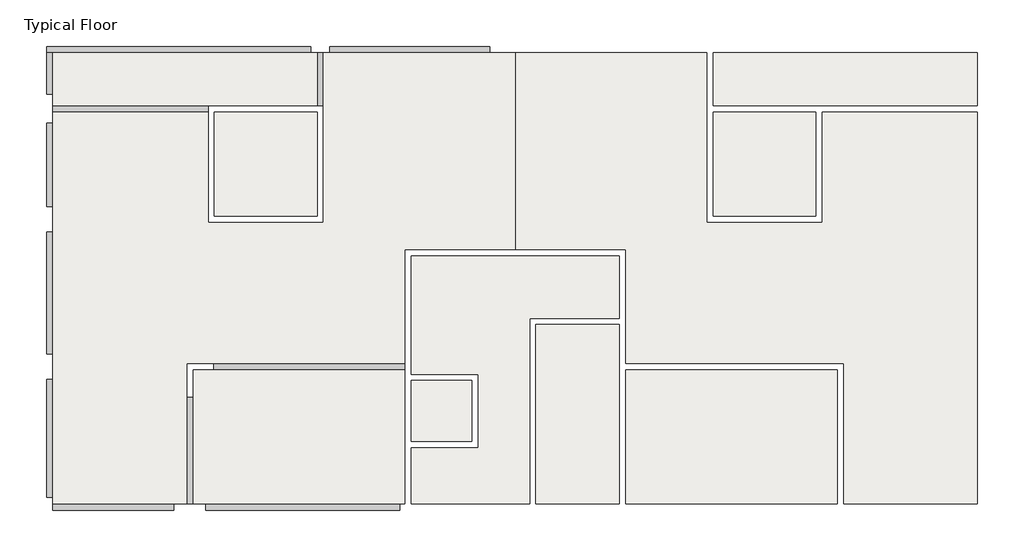
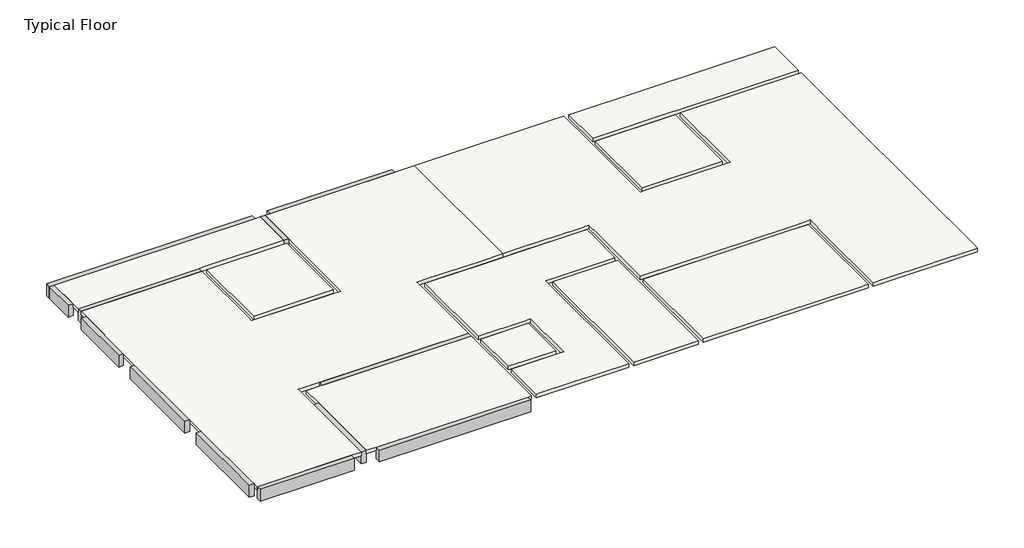
# One storey: 12 beams, 11 slabs.
"""IFC4 building model written with IfcOpenShell, lengths in millimetres."""

from ifc_helpers import new_model, si_unit, frame, origin, place, context, project, spatial, polyline, outline, extrude, faceted_brep, element, save

model = new_model("IFC4")

# Units and contexts
model_context = context("Model", 3, world=origin())
ifc_project = project(units=[si_unit("LENGTHUNIT", "METRE", prefix="MILLI")], contexts=[model_context])

# Site, building, storey
site = spatial("IfcSite", under=ifc_project)
building = spatial("IfcBuilding", under=site)
storey = spatial("IfcBuildingStorey", under=building, Name="Typical Floor", Elevation=3000.0)

# Beams
placement = place(None, origin())
element("IfcBeam", 1, ObjectType="Concrete Rectengular Beam : 20/50", at=placement, inside=storey, context=model_context, shape_type="SweptSolid", body=[
    extrude(outline(polyline([(-9297.7826138, 4182.4555068), (-9297.7826138, 4382.4555068), (-4303.3703529, 4382.4555068), (-4303.3703529, 4182.4555068), (-9297.7826138, 4182.4555068)])), frame((0.0, 0.0, 2500.0), z_axis=(0.0, 0.0, 1.0), x_axis=(1.0, 0.0, 0.0)), (0.0, 0.0, 1.0), 500.0),
])
element("IfcBeam", 2, ObjectType="Concrete Rectengular Beam : 20/50", at=placement, inside=storey, context=model_context, shape_type="Brep", body=[
    faceted_brep([(-18150.6144474, 4382.4555068, 3000.0), (-18150.6144474, 4182.4555068, 3000.0), (-17950.6144474, 4182.4555068, 3000.0), (-9897.7826138, 4182.4555068, 3000.0), (-9897.7826138, 4382.4555068, 3000.0), (-18150.6144474, 4182.4555068, 2500.0), (-17950.6144474, 4182.4555068, 2500.0), (-9897.7826138, 4182.4555068, 2500.0), (-18150.6144474, 4382.4555068, 2500.0), (-9897.7826138, 4382.4555068, 2500.0)], [[[0, 1, 2, 3, 4]], [[1, 5, 6, 7, 3, 2]], [[5, 8, 9, 7, 6]], [[8, 0, 4, 9]], [[4, 3, 7, 9]], [[1, 0, 8, 5]]]),
])
element("IfcBeam", 3, ObjectType="Concrete Rectengular Beam : 20/50", at=placement, inside=storey, context=model_context, shape_type="Brep", body=[
    faceted_brep([(-18150.6144474, 2884.276373, 3000.0), (-17950.6144474, 2884.276373, 3000.0), (-17950.6144474, 4182.4555068, 3000.0), (-18150.6144474, 4182.4555068, 3000.0), (-17950.6144474, 2884.276373, 2500.0), (-17950.6144474, 4182.4555068, 2500.0), (-17950.6144474, 4182.4555068, 2850.0), (-18150.6144474, 2884.276373, 2500.0), (-18150.6144474, 4182.4555068, 2500.0)], [[[0, 1, 2, 3]], [[1, 4, 5, 6, 2]], [[4, 7, 8, 5]], [[7, 0, 3, 8]], [[1, 0, 7, 4]], [[3, 2, 6, 5, 8]]]),
])
element("IfcBeam", 4, ObjectType="Concrete Rectengular Beam : 20/50", at=placement, inside=storey, context=model_context, shape_type="SweptSolid", body=[
    extrude(outline(polyline([(-17950.6144474, -618.260185), (-18150.6144474, -618.260185), (-18150.6144474, 1984.276373), (-17950.6144474, 1984.276373), (-17950.6144474, -618.260185)])), frame((0.0, 0.0, 2500.0), z_axis=(0.0, 0.0, 1.0), x_axis=(1.0, 0.0, 0.0)), (0.0, 0.0, 1.0), 500.0),
])
element("IfcBeam", 5, ObjectType="Concrete Rectengular Beam : 20/50", at=placement, inside=storey, context=model_context, shape_type="SweptSolid", body=[
    extrude(outline(polyline([(-18150.6144474, -1418.260185), (-17950.6144474, -1418.260185), (-17950.6144474, -5238.12942), (-18150.6144474, -5238.12942), (-18150.6144474, -1418.260185)])), frame((0.0, 0.0, 2500.0), z_axis=(0.0, 0.0, 1.0), x_axis=(1.0, 0.0, 0.0)), (0.0, 0.0, 1.0), 500.0),
])
element("IfcBeam", 6, ObjectType="Concrete Rectengular Beam : 20/50", at=placement, inside=storey, context=model_context, shape_type="SweptSolid", body=[
    extrude(outline(polyline([(-18150.6144474, -6038.12942), (-17950.6144474, -6038.12942), (-17950.6144474, -9718.1209836), (-18150.6144474, -9718.1209836), (-18150.6144474, -6038.12942)])), frame((0.0, 0.0, 2500.0), z_axis=(0.0, 0.0, 1.0), x_axis=(1.0, 0.0, 0.0)), (0.0, 0.0, 1.0), 500.0),
])
element("IfcBeam", 7, ObjectType="Concrete Rectengular Beam : 20/50", at=placement, inside=storey, context=model_context, shape_type="Brep", body=[
    faceted_brep([(-12922.2278424, -5538.12942, 3000.0), (-12922.2278424, -5738.12942, 3000.0), (-6954.5134912, -5738.12942, 3000.0), (-6954.5134912, -5538.12942, 3000.0), (-12922.2278424, -5538.12942, 2500.0), (-12922.2278424, -5538.12942, 2850.0), (-6954.5134912, -5538.12942, 2850.0), (-6954.5134912, -5538.12942, 2500.0), (-12922.2278424, -5738.12942, 2500.0), (-6954.5134912, -5738.12942, 2500.0), (-6954.5134912, -5738.12942, 2850.0)], [[[0, 1, 2, 3]], [[4, 5, 0, 3, 6, 7]], [[8, 4, 7, 9]], [[1, 8, 9, 10, 2]], [[1, 0, 5, 4, 8]], [[3, 2, 10, 9, 7, 6]]]),
])
element("IfcBeam", 8, ObjectType="Concrete Rectengular Beam : 20/50", at=placement, inside=storey, context=model_context, shape_type="Brep", body=[
    faceted_brep([(-13772.2278424, -9918.1209836, 3000.0), (-13572.2278424, -9918.1209836, 3000.0), (-13572.2278424, -6588.12942, 3000.0), (-13772.2278424, -6588.12942, 3000.0), (-13572.2278424, -9918.1209836, 2850.0), (-13572.2278424, -9918.1209836, 2500.0), (-13572.2278424, -6588.12942, 2500.0), (-13772.2278424, -9918.1209836, 2500.0), (-13772.2278424, -6588.12942, 2500.0), (-13772.2278424, -6588.12942, 2850.0), (-13772.2278424, -9918.1209836, 2850.0)], [[[0, 1, 2, 3]], [[1, 4, 5, 6, 2]], [[5, 7, 8, 6]], [[0, 3, 9, 8, 7, 10]], [[1, 0, 10, 7, 5, 4]], [[3, 2, 6, 8, 9]]]),
])
element("IfcBeam", 9, ObjectType="Concrete Rectengular Beam : 20/50", at=placement, inside=storey, context=model_context, shape_type="Brep", body=[
    faceted_brep([(-17950.6144474, -9918.1209836, 3000.0), (-17950.6144474, -10118.1209836, 3000.0), (-14171.4707466, -10118.1209836, 3000.0), (-14171.4707466, -9918.1209836, 3000.0), (-17950.6144474, -10118.1209836, 2500.0), (-14171.4707466, -10118.1209836, 2500.0), (-17950.6144474, -9918.1209836, 2500.0), (-14171.4707466, -9918.1209836, 2500.0), (-17950.6144474, -9918.1209836, 2850.0)], [[[0, 1, 2, 3]], [[1, 4, 5, 2]], [[4, 6, 7, 5]], [[6, 8, 0, 3, 7]], [[0, 8, 6, 4, 1]], [[3, 2, 5, 7]]]),
])
element("IfcBeam", 10, ObjectType="Concrete Rectengular Beam : 20/50", at=placement, inside=storey, context=model_context, shape_type="Brep", body=[
    faceted_brep([(-13104.0790143, 2334.276373, 3000.0), (-13104.0790143, 2534.276373, 3000.0), (-17950.6144474, 2534.276373, 3000.0), (-17950.6144474, 2334.276373, 3000.0), (-17950.6144474, 2534.276373, 2500.0), (-17950.6144474, 2534.276373, 2850.0), (-13104.0790143, 2534.276373, 2500.0), (-13104.0790143, 2334.276373, 2500.0), (-17950.6144474, 2334.276373, 2500.0), (-17950.6144474, 2334.276373, 2850.0), (-13104.0790143, 2334.276373, 2850.0)], [[[0, 1, 2, 3]], [[4, 5, 2, 1, 6]], [[6, 7, 8, 4]], [[0, 3, 9, 8, 7, 10]], [[2, 5, 4, 8, 9, 3]], [[1, 0, 10, 7, 6]]]),
])
element("IfcBeam", 11, ObjectType="Concrete Rectengular Beam : 20/50", at=placement, inside=storey, context=model_context, shape_type="Brep", body=[
    faceted_brep([(-9697.7826138, 2534.276373, 3000.0), (-9497.7826138, 2534.276373, 3000.0), (-9497.7826138, 4182.4555068, 3000.0), (-9697.7826138, 4182.4555068, 3000.0), (-9497.7826138, 2534.276373, 2850.0), (-9497.7826138, 2534.276373, 2500.0), (-9497.7826138, 4182.4555068, 2500.0), (-9497.7826138, 4182.4555068, 2850.0), (-9697.7826138, 2534.276373, 2500.0), (-9697.7826138, 4182.4555068, 2500.0), (-9697.7826138, 4182.4555068, 2850.0), (-9697.7826138, 2534.276373, 2850.0)], [[[0, 1, 2, 3]], [[2, 1, 4, 5, 6, 7]], [[5, 8, 9, 6]], [[3, 10, 9, 8, 11, 0]], [[9, 10, 3, 2, 7, 6]], [[1, 0, 11, 8, 5, 4]]]),
])
element("IfcBeam", 12, ObjectType="Concrete Rectengular Beam : 20/50", at=placement, inside=storey, context=model_context, shape_type="SweptSolid", body=[
    extrude(outline(polyline([(-13171.4707466, -10118.1209836), (-13171.4707466, -9918.1209836), (-7104.2111853, -9918.1209836), (-7104.2111853, -10118.1209836), (-13171.4707466, -10118.1209836)])), frame((0.0, 0.0, 2500.0), z_axis=(0.0, 0.0, 1.0), x_axis=(1.0, 0.0, 0.0)), (0.0, 0.0, 1.0), 500.0),
])

# Slabs
element("IfcSlab", 13, ObjectType="15", at=placement, inside=storey, context=model_context, shape_type="Brep", body=[
    faceted_brep([(10943.8737416, 4182.4555068, 2850.0), (10943.8737416, 2534.276373, 2850.0), (2691.0419081, 2534.276373, 2850.0), (2691.0419081, 4182.4555068, 2850.0), (10943.8737416, 4182.4555068, 3000.0), (2891.0419081, 4182.4555068, 3000.0), (2691.0419081, 4182.4555068, 3000.0), (2691.0419081, 2534.276373, 3000.0), (5897.3383085, 2534.276373, 3000.0), (6097.3383085, 2534.276373, 3000.0), (10943.8737416, 2534.276373, 3000.0), (10943.8737416, 2884.276373, 3000.0)], [[[0, 1, 2, 3]], [[4, 5, 6, 7, 8, 9, 10, 11]], [[1, 0, 4, 11, 10]], [[2, 1, 10, 9, 8, 7]], [[3, 2, 7, 6]], [[0, 3, 6, 5, 4]]]),
])
element("IfcSlab", 14, ObjectType="15", at=placement, inside=storey, context=model_context, shape_type="SweptSolid", body=[
    extrude(outline(polyline([(5897.3383085, 2334.276373), (5897.3383085, -917.4123222), (2691.0419081, -917.4123222), (2691.0419081, 2334.276373), (5897.3383085, 2334.276373)])), frame((0.0, 0.0, 2850.0), z_axis=(0.0, 0.0, 1.0), x_axis=(1.0, 0.0, 0.0)), (0.0, 0.0, 1.0), 150.0),
])
element("IfcSlab", 15, ObjectType="15", at=placement, inside=storey, context=model_context, shape_type="Brep", body=[
    faceted_brep([(6565.4871367, -5738.12942, 2850.0), (6565.4871367, -9918.1209836, 2850.0), (-55.6186656, -9918.1209836, 2850.0), (-55.6186656, -5738.12942, 2850.0), (6565.4871367, -5738.12942, 3000.0), (5915.4871367, -5738.12942, 3000.0), (-55.6186656, -5738.12942, 3000.0), (-55.6186656, -9918.1209836, 3000.0), (6164.7300408, -9918.1209836, 3000.0), (6565.4871367, -9918.1209836, 3000.0), (6565.4871367, -6588.12942, 3000.0)], [[[0, 1, 2, 3]], [[4, 5, 6, 7, 8, 9, 10]], [[1, 0, 4, 10, 9]], [[2, 1, 9, 8, 7]], [[3, 2, 7, 6]], [[0, 3, 6, 5, 4]]]),
])
element("IfcSlab", 16, ObjectType="15", at=placement, inside=storey, context=model_context, shape_type="Brep", body=[
    faceted_brep([(6097.3383085, 2334.276373, 2850.0), (10943.8737416, 2334.276373, 2850.0), (10943.8737416, -9918.1209836, 2850.0), (6765.4871367, -9918.1209836, 2850.0), (6765.4871367, -6588.12942, 2850.0), (6765.4871367, -5538.12942, 2850.0), (6565.4871367, -5538.12942, 2850.0), (5915.4871367, -5538.12942, 2850.0), (-55.6186656, -5538.12942, 2850.0), (-55.6186656, -4117.6485427, 2850.0), (-55.6186656, -2568.3192401, 2850.0), (-55.6186656, -1968.3192401, 2850.0), (-455.6186656, -1968.3192401, 2850.0), (-2804.4614665, -1968.3192401, 2850.0), (-3503.3835189, -1968.3192401, 2850.0), (-3503.3835189, 4182.4555068, 2850.0), (2491.0419081, 4182.4555068, 2850.0), (2491.0419081, 2534.276373, 2850.0), (2491.0419081, -1117.4123222, 2850.0), (2691.0419081, -1117.4123222, 2850.0), (6097.3383085, -1117.4123222, 2850.0), (6097.3383085, -917.4123222, 2850.0), (10943.8737416, 2334.276373, 3000.0), (6097.3383085, 2334.276373, 3000.0), (6097.3383085, -917.4123222, 3000.0), (6097.3383085, -1117.4123222, 3000.0), (2691.0419081, -1117.4123222, 3000.0), (2491.0419081, -1117.4123222, 3000.0), (2491.0419081, 2534.276373, 3000.0), (2491.0419081, 4182.4555068, 3000.0), (2291.0419081, 4182.4555068, 3000.0), (-2903.3703529, 4182.4555068, 3000.0), (-3503.3835189, 4182.4555068, 3000.0), (-3503.3835189, -1968.3192401, 3000.0), (-2804.4614665, -1968.3192401, 3000.0), (-455.6186656, -1968.3192401, 3000.0), (-55.6186656, -1968.3192401, 3000.0), (-55.6186656, -2568.3192401, 3000.0), (-55.6186656, -4117.6485427, 3000.0), (-55.6186656, -5538.12942, 3000.0), (5915.4871367, -5538.12942, 3000.0), (6565.4871367, -5538.12942, 3000.0), (6765.4871367, -5538.12942, 3000.0), (6765.4871367, -6588.12942, 3000.0), (6765.4871367, -9918.1209836, 3000.0), (7164.7300408, -9918.1209836, 3000.0), (10943.8737416, -9918.1209836, 3000.0), (10943.8737416, -9718.1209836, 3000.0), (10943.8737416, -6038.12942, 3000.0), (10943.8737416, -5238.12942, 3000.0), (10943.8737416, -1418.260185, 3000.0), (10943.8737416, -618.260185, 3000.0), (10943.8737416, 1984.276373, 3000.0)], [[[0, 1, 2, 3, 4, 5, 6, 7, 8, 9, 10, 11, 12, 13, 14, 15, 16, 17, 18, 19, 20, 21]], [[22, 23, 24, 25, 26, 27, 28, 29, 30, 31, 32, 33, 34, 35, 36, 37, 38, 39, 40, 41, 42, 43, 44, 45, 46, 47, 48, 49, 50, 51, 52]], [[27, 18, 17, 16, 29, 28]], [[18, 27, 26, 25, 20, 19]], [[20, 25, 24, 23, 0, 21]], [[1, 0, 23, 22]], [[2, 1, 22, 52, 51, 50, 49, 48, 47, 46]], [[3, 2, 46, 45, 44]], [[3, 44, 43, 42, 5, 4]], [[5, 42, 41, 40, 39, 8, 7, 6]], [[8, 39, 38, 37, 36, 11, 10, 9]], [[11, 36, 35, 34, 33, 14, 13, 12]], [[15, 14, 33, 32]], [[16, 15, 32, 31, 30, 29]]]),
])
element("IfcSlab", 17, ObjectType="15", at=placement, inside=storey, context=model_context, shape_type="SweptSolid", body=[
    extrude(outline(polyline([(-255.6186656, -4317.6485427), (-255.6186656, -9918.1209836), (-2855.8548861, -9918.1209836), (-2855.8548861, -4317.6485427), (-255.6186656, -4317.6485427)])), frame((0.0, 0.0, 2850.0), z_axis=(0.0, 0.0, 1.0), x_axis=(1.0, 0.0, 0.0)), (0.0, 0.0, 1.0), 150.0),
])
element("IfcSlab", 18, ObjectType="15", at=placement, inside=storey, context=model_context, shape_type="SweptSolid", body=[
    extrude(outline(polyline([(-4854.8818827, -6069.1600725), (-4854.8818827, -7968.791681), (-6754.8818827, -7968.791681), (-6754.8818827, -6069.1600725), (-4854.8818827, -6069.1600725)])), frame((0.0, 0.0, 2850.0), z_axis=(0.0, 0.0, 1.0), x_axis=(1.0, 0.0, 0.0)), (0.0, 0.0, 1.0), 150.0),
])
element("IfcSlab", 19, ObjectType="15", at=placement, inside=storey, context=model_context, shape_type="Brep", body=[
    faceted_brep([(-6754.8818827, -8168.791681, 2850.0), (-4654.8818827, -8168.791681, 2850.0), (-4654.8818827, -7968.791681, 2850.0), (-4654.8818827, -5869.1600725, 2850.0), (-4854.8818827, -5869.1600725, 2850.0), (-6754.5134912, -5869.1600725, 2850.0), (-6754.5134912, -2568.3192401, 2850.0), (-6754.5134912, -2168.3192401, 2850.0), (-6554.5134912, -2168.3192401, 2850.0), (-455.6186656, -2168.3192401, 2850.0), (-255.6186656, -2168.3192401, 2850.0), (-255.6186656, -2568.3192401, 2850.0), (-255.6186656, -4117.6485427, 2850.0), (-2855.8548861, -4117.6485427, 2850.0), (-3055.8548861, -4117.6485427, 2850.0), (-3055.8548861, -9918.1209836, 2850.0), (-6754.8818827, -9918.1209836, 2850.0), (-4654.8818827, -8168.791681, 3000.0), (-6754.8818827, -8168.791681, 3000.0), (-6754.8818827, -9918.1209836, 3000.0), (-6604.2111853, -9918.1209836, 3000.0), (-3055.8548861, -9918.1209836, 3000.0), (-3055.8548861, -4117.6485427, 3000.0), (-2855.8548861, -4117.6485427, 3000.0), (-255.6186656, -4117.6485427, 3000.0), (-255.6186656, -2568.3192401, 3000.0), (-255.6186656, -2168.3192401, 3000.0), (-455.6186656, -2168.3192401, 3000.0), (-2804.4614665, -2168.3192401, 3000.0), (-4404.4614665, -2168.3192401, 3000.0), (-6554.5134912, -2168.3192401, 3000.0), (-6754.5134912, -2168.3192401, 3000.0), (-6754.5134912, -2568.3192401, 3000.0), (-6754.5134912, -5869.1600725, 3000.0), (-4854.8818827, -5869.1600725, 3000.0), (-4654.8818827, -5869.1600725, 3000.0), (-4654.8818827, -7968.791681, 3000.0)], [[[0, 1, 2, 3, 4, 5, 6, 7, 8, 9, 10, 11, 12, 13, 14, 15, 16]], [[17, 18, 19, 20, 21, 22, 23, 24, 25, 26, 27, 28, 29, 30, 31, 32, 33, 34, 35, 36]], [[1, 0, 18, 17]], [[1, 17, 36, 35, 3, 2]], [[3, 35, 34, 33, 5, 4]], [[5, 33, 32, 31, 7, 6]], [[7, 31, 30, 29, 28, 27, 26, 10, 9, 8]], [[10, 26, 25, 24, 12, 11]], [[12, 24, 23, 22, 14, 13]], [[15, 14, 22, 21]], [[16, 15, 21, 20, 19]], [[0, 16, 19, 18]]]),
])
element("IfcSlab", 20, ObjectType="15", at=placement, inside=storey, context=model_context, shape_type="Brep", body=[
    faceted_brep([(-17950.6144474, 4182.4555068, 2850.0), (-9697.7826138, 4182.4555068, 2850.0), (-9697.7826138, 2534.276373, 2850.0), (-17950.6144474, 2534.276373, 2850.0), (-17950.6144474, 4182.4555068, 3000.0), (-17950.6144474, 2884.276373, 3000.0), (-17950.6144474, 2534.276373, 3000.0), (-13104.0790143, 2534.276373, 3000.0), (-12904.0790143, 2534.276373, 3000.0), (-9697.7826138, 2534.276373, 3000.0), (-9697.7826138, 4182.4555068, 3000.0), (-9897.7826138, 4182.4555068, 3000.0)], [[[0, 1, 2, 3]], [[4, 5, 6, 7, 8, 9, 10, 11]], [[0, 3, 6, 5, 4]], [[3, 2, 9, 8, 7, 6]], [[2, 1, 10, 9]], [[1, 0, 4, 11, 10]]]),
])
element("IfcSlab", 21, ObjectType="15", at=placement, inside=storey, context=model_context, shape_type="SweptSolid", body=[
    extrude(outline(polyline([(-12904.0790143, 2334.276373), (-9697.7826138, 2334.276373), (-9697.7826138, -917.4123222), (-12904.0790143, -917.4123222), (-12904.0790143, 2334.276373)])), frame((0.0, 0.0, 2850.0), z_axis=(0.0, 0.0, 1.0), x_axis=(1.0, 0.0, 0.0)), (0.0, 0.0, 1.0), 150.0),
])
element("IfcSlab", 22, ObjectType="15", at=placement, inside=storey, context=model_context, shape_type="Brep", body=[
    faceted_brep([(-13572.2278424, -9918.1209836, 2850.0), (-13572.2278424, -5738.12942, 2850.0), (-6954.5134912, -5738.12942, 2850.0), (-6953.6220402, -5738.12942, 2850.0), (-6953.6220402, -5869.1600725, 2850.0), (-6954.5134912, -5869.1600725, 2850.0), (-6954.8818827, -5869.1600725, 2850.0), (-6954.8818827, -8168.791681, 2850.0), (-6953.6220402, -8168.791681, 2850.0), (-6953.6220402, -9918.1209836, 2850.0), (-6954.8818827, -9918.1209836, 2850.0), (-13572.2278424, -5738.12942, 3000.0), (-13572.2278424, -6588.12942, 3000.0), (-13572.2278424, -9918.1209836, 3000.0), (-13171.4707466, -9918.1209836, 3000.0), (-7104.2111853, -9918.1209836, 3000.0), (-6953.6220402, -9918.1209836, 3000.0), (-6953.6220402, -8168.791681, 3000.0), (-6954.8818827, -8168.791681, 3000.0), (-6954.8818827, -7968.791681, 3000.0), (-6954.8818827, -6069.1600725, 3000.0), (-6954.8818827, -5869.1600725, 3000.0), (-6953.6220402, -5869.1600725, 3000.0), (-6953.6220402, -5738.12942, 3000.0), (-6954.5134912, -5738.12942, 3000.0), (-12922.2278424, -5738.12942, 3000.0)], [[[0, 1, 2, 3, 4, 5, 6, 7, 8, 9, 10]], [[11, 12, 13, 14, 15, 16, 17, 18, 19, 20, 21, 22, 23, 24, 25]], [[1, 0, 13, 12, 11]], [[0, 10, 9, 16, 15, 14, 13]], [[16, 9, 8, 17]], [[3, 23, 22, 4]], [[3, 2, 1, 11, 25, 24, 23]], [[7, 18, 17, 8]], [[18, 7, 6, 21, 20, 19]], [[21, 6, 5, 4, 22]]]),
])
element("IfcSlab", 23, ObjectType="15", at=placement, inside=storey, context=model_context, shape_type="Brep", body=[
    faceted_brep([(-17950.6144474, 2334.276373, 2850.0), (-13104.0790143, 2334.276373, 2850.0), (-13104.0790143, -917.4123222, 2850.0), (-13104.0790143, -1117.4123222, 2850.0), (-9697.7826138, -1117.4123222, 2850.0), (-9497.7826138, -1117.4123222, 2850.0), (-9497.7826138, 2534.276373, 2850.0), (-9497.7826138, 4182.4555068, 2850.0), (-3703.3703529, 4182.4555068, 2850.0), (-3503.3703529, 4182.4555068, 2850.0), (-3503.3703529, -1968.3192401, 2850.0), (-3703.3703529, -1968.3192401, 2850.0), (-6954.5134912, -1968.3192401, 2850.0), (-6954.5134912, -2568.3192401, 2850.0), (-6951.1220402, -2568.3192401, 2850.0), (-6951.1220402, -5538.12942, 2850.0), (-6954.5134912, -5538.12942, 2850.0), (-12922.2278424, -5538.12942, 2850.0), (-13572.2278424, -5538.12942, 2850.0), (-13772.2278424, -5538.12942, 2850.0), (-13772.2278424, -6588.12942, 2850.0), (-13772.2278424, -9918.1209836, 2850.0), (-17950.6144474, -9918.1209836, 2850.0), (-13104.0790143, 2334.276373, 3000.0), (-17950.6144474, 2334.276373, 3000.0), (-17950.6144474, 1984.276373, 3000.0), (-17950.6144474, -618.260185, 3000.0), (-17950.6144474, -1418.260185, 3000.0), (-17950.6144474, -5238.12942, 3000.0), (-17950.6144474, -6038.12942, 3000.0), (-17950.6144474, -9718.1209836, 3000.0), (-17950.6144474, -9918.1209836, 3000.0), (-14171.4707466, -9918.1209836, 3000.0), (-13772.2278424, -9918.1209836, 3000.0), (-13772.2278424, -6588.12942, 3000.0), (-13772.2278424, -5538.12942, 3000.0), (-13572.2278424, -5538.12942, 3000.0), (-12922.2278424, -5538.12942, 3000.0), (-6954.5134912, -5538.12942, 3000.0), (-6951.1220402, -5538.12942, 3000.0), (-6951.1220402, -2568.3192401, 3000.0), (-6954.5134912, -2568.3192401, 3000.0), (-6954.5134912, -1968.3192401, 3000.0), (-6554.5134912, -1968.3192401, 3000.0), (-4404.4614665, -1968.3192401, 3000.0), (-3503.3703529, -1968.3192401, 3000.0), (-3503.3703529, 4182.4555068, 3000.0), (-4303.3703529, 4182.4555068, 3000.0), (-9297.7826138, 4182.4555068, 3000.0), (-9497.7826138, 4182.4555068, 3000.0), (-9497.7826138, 2534.276373, 3000.0), (-9497.7826138, -1117.4123222, 3000.0), (-9697.7826138, -1117.4123222, 3000.0), (-13104.0790143, -1117.4123222, 3000.0), (-13104.0790143, -917.4123222, 3000.0)], [[[0, 1, 2, 3, 4, 5, 6, 7, 8, 9, 10, 11, 12, 13, 14, 15, 16, 17, 18, 19, 20, 21, 22]], [[23, 24, 25, 26, 27, 28, 29, 30, 31, 32, 33, 34, 35, 36, 37, 38, 39, 40, 41, 42, 43, 44, 45, 46, 47, 48, 49, 50, 51, 52, 53, 54]], [[5, 51, 50, 49, 7, 6]], [[3, 53, 52, 51, 5, 4]], [[1, 23, 54, 53, 3, 2]], [[1, 0, 24, 23]], [[0, 22, 31, 30, 29, 28, 27, 26, 25, 24]], [[22, 21, 33, 32, 31]], [[19, 35, 34, 33, 21, 20]], [[15, 39, 38, 37, 36, 35, 19, 18, 17, 16]], [[39, 15, 14, 40]], [[10, 45, 44, 43, 42, 12, 11]], [[10, 9, 46, 45]], [[9, 8, 7, 49, 48, 47, 46]], [[13, 41, 40, 14]], [[41, 13, 12, 42]]]),
])

save(model, "model.ifc")

# Revit data of these elements
# Type "Concrete Rectengular Beam : 20/50"
#   Length [instance default] = 152.4 cm
#   b = 20 cm
#   h = 50 cm
#   Structural Material [instance default] = Concrete
#   Assembly Code = ""
# Type "15"
#   Function = 0
#   Layers, outside or top first: 15 cm "Concrete" (function 1)
# Element 1 (IfcBeam, "Concrete Rectengular Beam : 20/50")
#   Comments = ""
#   Mark = "B20"
#   SOFiSTiK_AMG_Comments = ""
#   SOFiSTiK_AMG_Scheduled = yes
#   SOFiSTiK_AMG_Adjusted = yes
#   Structural Material = Concrete
#   Phase Created = New Construction
#   Materials on its faces: "Concrete"
# Element 2 (IfcBeam, "Concrete Rectengular Beam : 20/50")
#   Comments = ""
#   Mark = "B21"
#   SOFiSTiK_AMG_Comments = ""
#   SOFiSTiK_AMG_Scheduled = yes
#   SOFiSTiK_AMG_Adjusted = yes
#   Structural Material = Concrete
#   Phase Created = New Construction
#   Materials on its faces: "Concrete"
# Element 3 (IfcBeam, "Concrete Rectengular Beam : 20/50")
#   Comments = ""
#   Mark = "B22"
#   SOFiSTiK_AMG_Comments = ""
#   SOFiSTiK_AMG_Scheduled = yes
#   SOFiSTiK_AMG_Adjusted = yes
#   Structural Material = Concrete
#   Phase Created = New Construction
#   Materials on its faces: "Concrete"
# Element 4 (IfcBeam, "Concrete Rectengular Beam : 20/50")
#   Comments = ""
#   Mark = "B23"
#   SOFiSTiK_AMG_Comments = ""
#   SOFiSTiK_AMG_Scheduled = yes
#   SOFiSTiK_AMG_Adjusted = yes
#   Structural Material = Concrete
#   Phase Created = New Construction
#   Materials on its faces: "Concrete"
# Element 5 (IfcBeam, "Concrete Rectengular Beam : 20/50")
#   Comments = ""
#   Mark = "B24"
#   SOFiSTiK_AMG_Comments = ""
#   SOFiSTiK_AMG_Scheduled = yes
#   SOFiSTiK_AMG_Adjusted = yes
#   Structural Material = Concrete
#   Phase Created = New Construction
#   Materials on its faces: "Concrete"
# Element 6 (IfcBeam, "Concrete Rectengular Beam : 20/50")
#   Comments = ""
#   Mark = "B25"
#   SOFiSTiK_AMG_Comments = ""
#   SOFiSTiK_AMG_Scheduled = yes
#   SOFiSTiK_AMG_Adjusted = yes
#   Structural Material = Concrete
#   Phase Created = New Construction
#   Materials on its faces: "Concrete"
# Element 7 (IfcBeam, "Concrete Rectengular Beam : 20/50")
#   Comments = ""
#   Mark = "B26"
#   SOFiSTiK_AMG_Comments = ""
#   SOFiSTiK_AMG_Scheduled = yes
#   SOFiSTiK_AMG_Adjusted = yes
#   Structural Material = Concrete
#   Phase Created = New Construction
#   Materials on its faces: "Concrete"
# Element 8 (IfcBeam, "Concrete Rectengular Beam : 20/50")
#   Comments = ""
#   Mark = "B27"
#   SOFiSTiK_AMG_Comments = ""
#   SOFiSTiK_AMG_Scheduled = yes
#   SOFiSTiK_AMG_Adjusted = yes
#   Structural Material = Concrete
#   Phase Created = New Construction
#   Materials on its faces: "Concrete"
# Element 9 (IfcBeam, "Concrete Rectengular Beam : 20/50")
#   Comments = ""
#   Mark = "B28"
#   SOFiSTiK_AMG_Comments = ""
#   SOFiSTiK_AMG_Scheduled = yes
#   SOFiSTiK_AMG_Adjusted = yes
#   Structural Material = Concrete
#   Phase Created = New Construction
#   Materials on its faces: "Concrete"
# Element 10 (IfcBeam, "Concrete Rectengular Beam : 20/50")
#   Comments = ""
#   Mark = "B29"
#   SOFiSTiK_AMG_Comments = ""
#   SOFiSTiK_AMG_Scheduled = yes
#   SOFiSTiK_AMG_Adjusted = yes
#   Structural Material = Concrete
#   Phase Created = New Construction
#   Materials on its faces: "Concrete"
# Element 11 (IfcBeam, "Concrete Rectengular Beam : 20/50")
#   Comments = ""
#   Mark = "B30"
#   SOFiSTiK_AMG_Comments = ""
#   SOFiSTiK_AMG_Scheduled = yes
#   SOFiSTiK_AMG_Adjusted = yes
#   Structural Material = Concrete
#   Phase Created = New Construction
#   Materials on its faces: "Concrete"
# Element 12 (IfcBeam, "Concrete Rectengular Beam : 20/50")
#   Comments = ""
#   Mark = "B31"
#   SOFiSTiK_AMG_Comments = ""
#   SOFiSTiK_AMG_Scheduled = yes
#   SOFiSTiK_AMG_Adjusted = yes
#   Structural Material = Concrete
#   Phase Created = New Construction
#   Materials on its faces: "Concrete"
# Element 13 (IfcSlab, "15")
#   Mark = "S1"
#   SOFiSTiK_AMG_Comments = ""
#   Height Offset From Level = 0 cm
#   built-in parameter 1001954 = 1
#   SOFiSTiK_AMG_Scheduled = yes
#   SOFiSTiK_AMG_Adjusted = yes
#   Phase Created = New Construction
#   Materials on its faces: "Concrete"
# Element 14 (IfcSlab, "15")
#   Mark = "S2"
#   SOFiSTiK_AMG_Comments = ""
#   Height Offset From Level = 0 cm
#   built-in parameter 1001954 = 1
#   SOFiSTiK_AMG_Scheduled = yes
#   SOFiSTiK_AMG_Adjusted = yes
#   Phase Created = New Construction
#   Materials on its faces: "Concrete"
# Element 15 (IfcSlab, "15")
#   Mark = "S3"
#   SOFiSTiK_AMG_Comments = ""
#   Height Offset From Level = 0 cm
#   built-in parameter 1001954 = 1
#   SOFiSTiK_AMG_Scheduled = yes
#   SOFiSTiK_AMG_Adjusted = yes
#   Phase Created = New Construction
#   Materials on its faces: "Concrete"
# Element 16 (IfcSlab, "15")
#   Mark = "S4"
#   SOFiSTiK_AMG_Comments = ""
#   Height Offset From Level = 0 cm
#   built-in parameter 1001954 = 1
#   SOFiSTiK_AMG_Scheduled = yes
#   SOFiSTiK_AMG_Adjusted = yes
#   Phase Created = New Construction
#   Materials on its faces: "Concrete"
# Element 17 (IfcSlab, "15")
#   Mark = "S5"
#   SOFiSTiK_AMG_Comments = ""
#   Height Offset From Level = 0 cm
#   built-in parameter 1001954 = 1
#   SOFiSTiK_AMG_Scheduled = yes
#   SOFiSTiK_AMG_Adjusted = yes
#   Phase Created = New Construction
#   Materials on its faces: "Concrete"
# Element 18 (IfcSlab, "15")
#   Mark = "S6"
#   SOFiSTiK_AMG_Comments = ""
#   Height Offset From Level = 0 cm
#   built-in parameter 1001954 = 1
#   SOFiSTiK_AMG_Scheduled = yes
#   SOFiSTiK_AMG_Adjusted = yes
#   Phase Created = New Construction
#   Materials on its faces: "Concrete"
# Element 19 (IfcSlab, "15")
#   Mark = "S7"
#   SOFiSTiK_AMG_Comments = ""
#   built-in parameter 1001955 = 1.5708 (stored number, unit not read)
#   Height Offset From Level = 0 cm
#   built-in parameter 1001954 = 1
#   SOFiSTiK_AMG_Scheduled = yes
#   SOFiSTiK_AMG_Adjusted = yes
#   Phase Created = New Construction
#   Materials on its faces: "Concrete"
# Element 20 (IfcSlab, "15")
#   Mark = "S8"
#   SOFiSTiK_AMG_Comments = ""
#   built-in parameter 1001955 = 3.14159 (stored number, unit not read)
#   Height Offset From Level = 0 cm
#   built-in parameter 1001954 = 1
#   SOFiSTiK_AMG_Scheduled = yes
#   SOFiSTiK_AMG_Adjusted = yes
#   Phase Created = New Construction
#   Materials on its faces: "Concrete"
# Element 21 (IfcSlab, "15")
#   Mark = "S9"
#   SOFiSTiK_AMG_Comments = ""
#   built-in parameter 1001955 = 3.14159 (stored number, unit not read)
#   Height Offset From Level = 0 cm
#   built-in parameter 1001954 = 1
#   SOFiSTiK_AMG_Scheduled = yes
#   SOFiSTiK_AMG_Adjusted = yes
#   Phase Created = New Construction
#   Materials on its faces: "Concrete"
# Element 22 (IfcSlab, "15")
#   Mark = "S10"
#   SOFiSTiK_AMG_Comments = ""
#   built-in parameter 1001955 = 3.14159 (stored number, unit not read)
#   Height Offset From Level = 0 cm
#   built-in parameter 1001954 = 1
#   SOFiSTiK_AMG_Scheduled = yes
#   SOFiSTiK_AMG_Adjusted = yes
#   Phase Created = New Construction
#   Materials on its faces: "Concrete"
# Element 23 (IfcSlab, "15")
#   Mark = "S11"
#   SOFiSTiK_AMG_Comments = ""
#   built-in parameter 1001955 = 3.14159 (stored number, unit not read)
#   Height Offset From Level = 0 cm
#   built-in parameter 1001954 = 1
#   SOFiSTiK_AMG_Scheduled = yes
#   SOFiSTiK_AMG_Adjusted = yes
#   Phase Created = New Construction
#   Materials on its faces: "Concrete"
# Materials
#   "Concrete": class "Concrete", colour RGB 192 192 192, transparency 0, Keynote = "01000", Description = "Cast-in-place concrete", Cost = 0
